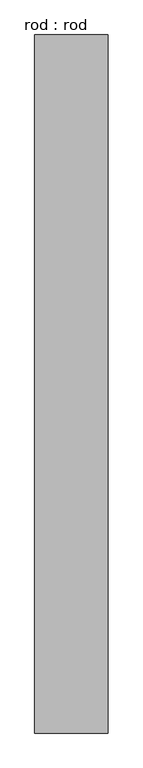
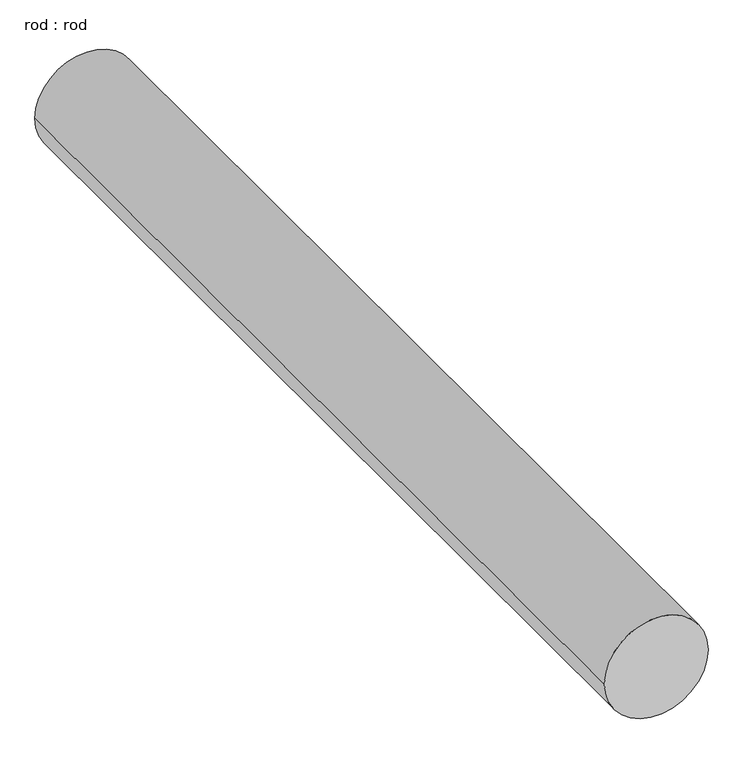
"""IFC4 building model written with IfcOpenShell, lengths in millimetres: proxy geometry, rod : rod."""

from ifc_helpers import new_model, si_unit, point, frame, frame_2d, origin, place, context, project, spatial, circle_curve, trimmed, segment, composite_curve, outline, extrude, source, transform, mapped, element, save


def rod_rod_dc578d62(model_context):
    return source(origin(), model_context, "Body", "SweptSolid", [
        extrude(outline(composite_curve([segment(trimmed(circle_curve(frame_2d((0.0108462, 0.0)), 200.0), [point((0.0108462, 200.0))], [point((0.0108462, -200.0))], False, "CARTESIAN"), True, "CONTINUOUS"), segment(trimmed(circle_curve(frame_2d((0.0108462, 0.0)), 200.0), [point((0.0108462, -200.0))], [point((0.0108462, 200.0))], False, "CARTESIAN"), True, "CONTINUOUS")], self_intersect=False)), frame((0.0, 2190.3370179, 0.0), z_axis=(0.0, 1.0, 0.0), x_axis=(0.0, 0.0, 1.0)), (0.0, 0.0, 1.0), 3804.7831948),
    ])


if __name__ == "__main__":
    model = new_model("IFC4")
    model_context = context("Model", 3, world=origin())
    ifc_project = project(units=[si_unit("LENGTHUNIT", "METRE", prefix="MILLI")], contexts=[model_context])
    site = spatial("IfcSite", under=ifc_project)
    building = spatial("IfcBuilding", under=site)
    placement = place(None, origin())
    rod_rod_shape = rod_rod_dc578d62(model_context)
    element("IfcBuildingElementProxy", 1, Name="rod : rod", ObjectType="rod : rod", at=placement, inside=building, context=model_context, shape_type="MappedRepresentation", body=[
        mapped(rod_rod_shape, transform((0.0, 0.0, 0.0), x_axis=(1.0, 0.0, 0.0), y_axis=(0.0, 1.0, 0.0), z_axis=(0.0, 0.0, 1.0))),
    ])
    save(model, "model.ifc")

# Revit data of these elements
# Type "rod : rod"
#   Default Elevation = 0
